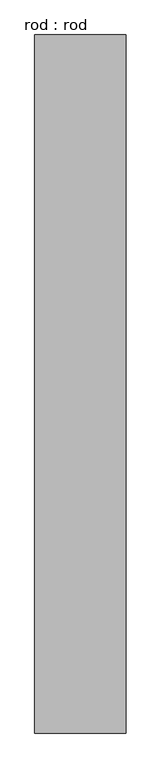
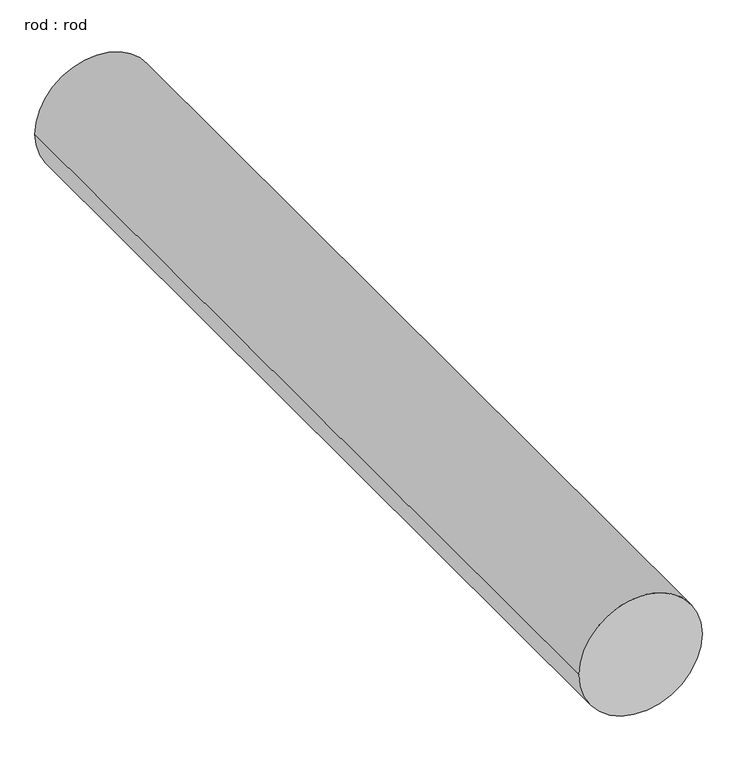
"""IFC4 building model written with IfcOpenShell, lengths in millimetres: proxy geometry, rod : rod."""

from ifc_helpers import new_model, si_unit, point, frame, frame_2d, origin, place, context, project, spatial, circle_curve, trimmed, segment, composite_curve, outline, extrude, source, transform, mapped, element, save


def rod_rod_4074fae5(model_context):
    return source(origin(), model_context, "Body", "SweptSolid", [
        extrude(outline(composite_curve([segment(trimmed(circle_curve(frame_2d((0.0108462, 0.0)), 200.0), [point((0.0108462, 200.0))], [point((0.0108462, -200.0))], False, "CARTESIAN"), True, "CONTINUOUS"), segment(trimmed(circle_curve(frame_2d((0.0108462, 0.0)), 200.0), [point((0.0108462, -200.0))], [point((0.0108462, 200.0))], False, "CARTESIAN"), True, "CONTINUOUS")], self_intersect=False)), frame((0.0, 2562.7286153, 0.0), z_axis=(0.0, 1.0, 0.0), x_axis=(0.0, 0.0, 1.0)), (0.0, 0.0, 1.0), 3060.0),
    ])


if __name__ == "__main__":
    model = new_model("IFC4")
    model_context = context("Model", 3, world=origin())
    ifc_project = project(units=[si_unit("LENGTHUNIT", "METRE", prefix="MILLI")], contexts=[model_context])
    site = spatial("IfcSite", under=ifc_project)
    building = spatial("IfcBuilding", under=site)
    placement = place(None, origin())
    rod_rod_shape = rod_rod_4074fae5(model_context)
    element("IfcBuildingElementProxy", 1, Name="rod : rod", ObjectType="rod : rod", at=placement, inside=building, context=model_context, shape_type="MappedRepresentation", body=[
        mapped(rod_rod_shape, transform((0.0, 0.0, 0.0), x_axis=(1.0, 0.0, 0.0), y_axis=(0.0, 1.0, 0.0), z_axis=(0.0, 0.0, 1.0))),
    ])
    save(model, "model.ifc")

# Revit data of these elements
# Type "rod : rod"
#   Default Elevation = 0
